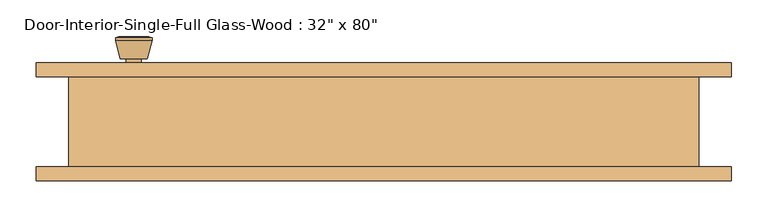
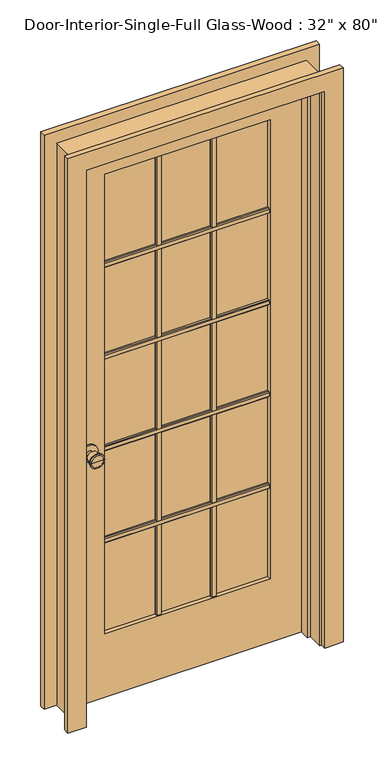
"""IFC4 building model written with IfcOpenShell, lengths in millimetres: door geometry."""

from ifc_helpers import new_model, si_unit, point, frame, frame_2d, origin, place, context, project, spatial, polyline, circle_curve, trimmed, segment, composite_curve, outline, extrude, faceted_brep, source, transform, mapped, element, save
from ifc_brep_helpers import plane_surface, cylinder_surface, revolved_surface, advanced_brep


def door_ad4706cc(model_context):
    return source(origin(), model_context, "Body", "SolidModel", [
        extrude(outline(polyline([(44.7675, 1586.23), (51.1175, 1586.23), (54.2925, 1583.055), (54.2925, 1570.355), (51.1175, 1567.18), (44.7675, 1567.18), (44.7675, 1586.23)])), frame((-285.75, 0.0, 0.0), z_axis=(1.0, 0.0, 0.0), x_axis=(0.0, 1.0, 0.0)), (0.0, 0.0, 1.0), 571.5),
        extrude(outline(polyline([(44.7675, 1249.9975), (51.1175, 1249.9975), (54.2925, 1246.8225), (54.2925, 1234.1225), (51.1175, 1230.9475), (44.7675, 1230.9475), (44.7675, 1249.9975)])), frame((-285.75, 0.0, 0.0), z_axis=(1.0, 0.0, 0.0), x_axis=(0.0, 1.0, 0.0)), (0.0, 0.0, 1.0), 571.5),
        extrude(outline(polyline([(44.7675, 913.765), (51.1175, 913.765), (54.2925, 910.59), (54.2925, 897.89), (51.1175, 894.715), (44.7675, 894.715), (44.7675, 913.765)])), frame((-285.75, 0.0, 0.0), z_axis=(1.0, 0.0, 0.0), x_axis=(0.0, 1.0, 0.0)), (0.0, 0.0, 1.0), 571.5),
        extrude(outline(polyline([(44.7675, 577.5325), (51.1175, 577.5325), (54.2925, 574.3575), (54.2925, 561.6575), (51.1175, 558.4825), (44.7675, 558.4825), (44.7675, 577.5325)])), frame((-285.75, 0.0, 0.0), z_axis=(1.0, 0.0, 0.0), x_axis=(0.0, 1.0, 0.0)), (0.0, 0.0, 1.0), 571.5),
        extrude(outline(polyline([(85.725, 44.7675), (85.725, 51.1175), (88.9, 54.2925), (101.6, 54.2925), (104.775, 51.1175), (104.775, 44.7675), (85.725, 44.7675)])), frame((0.0, 0.0, 231.775), z_axis=(0.0, 0.0, 1.0), x_axis=(1.0, 0.0, 0.0)), (0.0, 0.0, 1.0), 1681.1625),
        extrude(outline(polyline([(-104.775, 44.7675), (-104.775, 51.1175), (-101.6, 54.2925), (-88.9, 54.2925), (-85.725, 51.1175), (-85.725, 44.7675), (-104.775, 44.7675)])), frame((0.0, 0.0, 231.775), z_axis=(0.0, 0.0, 1.0), x_axis=(1.0, 0.0, 0.0)), (0.0, 0.0, 1.0), 1681.1625),
        extrude(outline(polyline([(37.7825, 1586.23), (37.7825, 1567.18), (31.4325, 1567.18), (28.2575, 1570.355), (28.2575, 1583.055), (31.4325, 1586.23), (37.7825, 1586.23)])), frame((-285.75, 0.0, 0.0), z_axis=(1.0, 0.0, 0.0), x_axis=(0.0, 1.0, 0.0)), (0.0, 0.0, 1.0), 571.5),
        extrude(outline(polyline([(37.7825, 1249.9975), (37.7825, 1230.9475), (31.4325, 1230.9475), (28.2575, 1234.1225), (28.2575, 1246.8225), (31.4325, 1249.9975), (37.7825, 1249.9975)])), frame((-285.75, 0.0, 0.0), z_axis=(1.0, 0.0, 0.0), x_axis=(0.0, 1.0, 0.0)), (0.0, 0.0, 1.0), 571.5),
        extrude(outline(polyline([(37.7825, 913.765), (37.7825, 894.715), (31.4325, 894.715), (28.2575, 897.89), (28.2575, 910.59), (31.4325, 913.765), (37.7825, 913.765)])), frame((-285.75, 0.0, 0.0), z_axis=(1.0, 0.0, 0.0), x_axis=(0.0, 1.0, 0.0)), (0.0, 0.0, 1.0), 571.5),
        extrude(outline(polyline([(37.7825, 577.5325), (37.7825, 558.4825), (31.4325, 558.4825), (28.2575, 561.6575), (28.2575, 574.3575), (31.4325, 577.5325), (37.7825, 577.5325)])), frame((-285.75, 0.0, 0.0), z_axis=(1.0, 0.0, 0.0), x_axis=(0.0, 1.0, 0.0)), (0.0, 0.0, 1.0), 571.5),
        extrude(outline(polyline([(85.725, 37.7825), (104.775, 37.7825), (104.775, 31.4325), (101.6, 28.2575), (88.9, 28.2575), (85.725, 31.4325), (85.725, 37.7825)])), frame((0.0, 0.0, 231.775), z_axis=(0.0, 0.0, 1.0), x_axis=(1.0, 0.0, 0.0)), (0.0, 0.0, 1.0), 1681.1625),
        extrude(outline(polyline([(-104.775, 37.7825), (-85.725, 37.7825), (-85.725, 31.4325), (-88.9, 28.2575), (-101.6, 28.2575), (-104.775, 31.4325), (-104.775, 37.7825)])), frame((0.0, 0.0, 231.775), z_axis=(0.0, 0.0, 1.0), x_axis=(1.0, 0.0, 0.0)), (0.0, 0.0, 1.0), 1681.1625),
        advanced_brep(
        [(-342.9, 17.8125, 914.4), (-332.9, 17.8125, 914.4), (-352.9, 17.8125, 914.4), (-322.4241324, -31.1875, 914.4), (-342.9, -31.1875, 914.4), (-363.3758676, -31.1875, 914.4), (-317.9, -29.3596319, 914.4), (-367.9, -29.3596319, 914.4), (-317.9, -25.8959537, 914.4), (-367.9, -25.8959537, 914.4), (-324.263764, -1.1875, 914.4), (-361.536236, -1.1875, 914.4), (-332.9, -1.1875, 914.4), (-352.9, -1.1875, 914.4)],
        [
            (0, 1),
            (1, 2, circle_curve(frame((-342.9, 17.8125, 914.4), z_axis=(0.0, 1.0, 0.0), x_axis=(-1.0, 0.0, 0.0)), 10.0)),
            (2, 0),
            (2, 1, circle_curve(frame((-342.9, 17.8125, 914.4), z_axis=(0.0, 1.0, 0.0), x_axis=(-1.0, 0.0, 0.0)), 10.0)),
            (3, 4),
            (4, 5),
            (5, 3, circle_curve(frame((-342.9, -31.1875, 914.4), z_axis=(0.0, -1.0, 0.0), x_axis=(-1.0, 0.0, 0.0)), 20.4758676)),
            (3, 5, circle_curve(frame((-342.9, -31.1875, 914.4), z_axis=(0.0, -1.0, 0.0), x_axis=(-1.0, 0.0, 0.0)), 20.4758676)),
            (6, 3),
            (5, 7),
            (7, 6, circle_curve(frame((-342.9, -29.3596319, 914.4), z_axis=(0.0, -1.0, 0.0), x_axis=(-1.0, 0.0, 0.0)), 25.0)),
            (6, 7, circle_curve(frame((-342.9, -29.3596319, 914.4), z_axis=(0.0, -1.0, 0.0), x_axis=(-1.0, 0.0, 0.0)), 25.0)),
            (8, 6),
            (7, 9),
            (9, 8, circle_curve(frame((-342.9, -25.8959537, 914.4), z_axis=(0.0, -1.0, 0.0), x_axis=(-1.0, 0.0, 0.0)), 25.0)),
            (8, 9, circle_curve(frame((-342.9, -25.8959537, 914.4), z_axis=(0.0, -1.0, 0.0), x_axis=(-1.0, 0.0, 0.0)), 25.0)),
            (10, 8),
            (9, 11),
            (11, 10, circle_curve(frame((-342.9, -1.1875, 914.4), z_axis=(0.0, -1.0, 0.0), x_axis=(-1.0, 0.0, 0.0)), 18.636236)),
            (10, 11, circle_curve(frame((-342.9, -1.1875, 914.4), z_axis=(0.0, -1.0, 0.0), x_axis=(-1.0, 0.0, 0.0)), 18.636236)),
            (12, 10),
            (11, 13),
            (13, 12, circle_curve(frame((-342.9, -1.1875, 914.4), z_axis=(0.0, -1.0, 0.0), x_axis=(-1.0, 0.0, 0.0)), 10.0)),
            (12, 13, circle_curve(frame((-342.9, -1.1875, 914.4), z_axis=(0.0, -1.0, 0.0), x_axis=(-1.0, 0.0, 0.0)), 10.0)),
            (1, 12),
            (13, 2),
        ],
        [
            plane_surface(frame((-342.9, 17.8125, 914.4), z_axis=(0.0, 1.0, 0.0), x_axis=(-1.0, 0.0, 0.0))),
            plane_surface(frame((-342.9, -31.1875, 914.4), z_axis=(0.0, -1.0, 0.0), x_axis=(-1.0, 0.0, 0.0))),
            revolved_surface(polyline([(-363.3758676, -31.1875, 914.4), (-367.9, -29.3596319, 914.4)]), (-342.9, 17.8125, 914.4), (0.0, 1.0, 0.0)),
            cylinder_surface(frame((-342.9, 17.8125, 914.4), z_axis=(0.0, 1.0, 0.0), x_axis=(-1.0, 0.0, 0.0)), 25.0),
            revolved_surface(polyline([(-367.9, -25.8959537, 914.4), (-361.536236, -1.1875, 914.4)]), (-342.9, 17.8125, 914.4), (0.0, 1.0, 0.0)),
            plane_surface(frame((-342.9, -1.1875, 914.4), z_axis=(0.0, 1.0, 0.0), x_axis=(-1.0, 0.0, 0.0))),
            cylinder_surface(frame((-342.9, 17.8125, 914.4), z_axis=(0.0, 1.0, 0.0), x_axis=(-1.0, 0.0, 0.0)), 10.0),
        ],
        [
            (0, [[1, 2, 3]]),
            (0, [[-3, 4, -1]]),
            (1, [[5, 6, 7]]),
            (1, [[-6, -5, 8]]),
            (2, [[9, -7, 10, 11]]),
            (2, [[-10, -8, -9, 12]]),
            (3, [[13, -11, 14, 15]]),
            (3, [[-14, -12, -13, 16]]),
            (4, [[17, -15, 18, 19]]),
            (4, [[-18, -16, -17, 20]]),
            (5, [[21, -19, 22, 23]]),
            (5, [[-22, -20, -21, 24]]),
            (6, [[25, -23, 26, -2]]),
            (6, [[-26, -24, -25, -4]]),
        ],
    ),
        extrude(outline(composite_curve([segment(trimmed(circle_curve(frame_2d((914.4, -342.9)), 30.0), [point((914.4, -372.9))], [point((914.4, -312.9))], False, "CARTESIAN"), True, "CONTINUOUS"), segment(trimmed(circle_curve(frame_2d((914.4, -342.9)), 30.0), [point((914.4, -312.9))], [point((914.4, -372.9))], False, "CARTESIAN"), True, "CONTINUOUS")], self_intersect=False)), frame((0.0, 17.8125, 0.0), z_axis=(0.0, 1.0, 0.0), x_axis=(0.0, 0.0, 1.0)), (0.0, 0.0, 1.0), 6.0),
        advanced_brep(
        [(-342.9, 64.7375, 914.4), (-352.9, 64.7375, 914.4), (-332.9, 64.7375, 914.4), (-322.4241324, 113.7375, 914.4), (-363.3758676, 113.7375, 914.4), (-342.9, 113.7375, 914.4), (-317.9, 111.9096319, 914.4), (-367.9, 111.9096319, 914.4), (-317.9, 108.4459537, 914.4), (-367.9, 108.4459537, 914.4), (-324.263764, 83.7375, 914.4), (-361.536236, 83.7375, 914.4), (-332.9, 83.7375, 914.4), (-352.9, 83.7375, 914.4)],
        [
            (0, 1),
            (1, 2, circle_curve(frame((-342.9, 64.7375, 914.4), z_axis=(0.0, -1.0, 0.0), x_axis=(-1.0, 0.0, 0.0)), 10.0)),
            (2, 0),
            (2, 1, circle_curve(frame((-342.9, 64.7375, 914.4), z_axis=(0.0, -1.0, 0.0), x_axis=(-1.0, 0.0, 0.0)), 10.0)),
            (3, 4, circle_curve(frame((-342.9, 113.7375, 914.4), z_axis=(0.0, 1.0, 0.0), x_axis=(-1.0, 0.0, 0.0)), 20.4758676)),
            (4, 5),
            (5, 3),
            (4, 3, circle_curve(frame((-342.9, 113.7375, 914.4), z_axis=(0.0, 1.0, 0.0), x_axis=(-1.0, 0.0, 0.0)), 20.4758676)),
            (6, 7, circle_curve(frame((-342.9, 111.9096319, 914.4), z_axis=(0.0, 1.0, 0.0), x_axis=(-1.0, 0.0, 0.0)), 25.0)),
            (7, 4),
            (3, 6),
            (7, 6, circle_curve(frame((-342.9, 111.9096319, 914.4), z_axis=(0.0, 1.0, 0.0), x_axis=(-1.0, 0.0, 0.0)), 25.0)),
            (8, 9, circle_curve(frame((-342.9, 108.4459537, 914.4), z_axis=(0.0, 1.0, 0.0), x_axis=(-1.0, 0.0, 0.0)), 25.0)),
            (9, 7),
            (6, 8),
            (9, 8, circle_curve(frame((-342.9, 108.4459537, 914.4), z_axis=(0.0, 1.0, 0.0), x_axis=(-1.0, 0.0, 0.0)), 25.0)),
            (10, 11, circle_curve(frame((-342.9, 83.7375, 914.4), z_axis=(0.0, 1.0, 0.0), x_axis=(-1.0, 0.0, 0.0)), 18.636236)),
            (11, 9),
            (8, 10),
            (11, 10, circle_curve(frame((-342.9, 83.7375, 914.4), z_axis=(0.0, 1.0, 0.0), x_axis=(-1.0, 0.0, 0.0)), 18.636236)),
            (12, 13, circle_curve(frame((-342.9, 83.7375, 914.4), z_axis=(0.0, 1.0, 0.0), x_axis=(-1.0, 0.0, 0.0)), 10.0)),
            (13, 11),
            (10, 12),
            (13, 12, circle_curve(frame((-342.9, 83.7375, 914.4), z_axis=(0.0, 1.0, 0.0), x_axis=(-1.0, 0.0, 0.0)), 10.0)),
            (1, 13),
            (12, 2),
        ],
        [
            plane_surface(frame((-342.9, 64.7375, 914.4), z_axis=(0.0, -1.0, 0.0), x_axis=(-1.0, 0.0, 0.0))),
            plane_surface(frame((-342.9, 113.7375, 914.4), z_axis=(0.0, 1.0, 0.0), x_axis=(-1.0, 0.0, 0.0))),
            revolved_surface(polyline([(-363.3758676, 113.7375, 914.4), (-367.9, 111.9096319, 914.4)]), (-342.9, 64.7375, 914.4), (0.0, -1.0, 0.0)),
            cylinder_surface(frame((-342.9, 64.7375, 914.4), z_axis=(0.0, -1.0, 0.0), x_axis=(-1.0, 0.0, 0.0)), 25.0),
            revolved_surface(polyline([(-367.9, 108.4459537, 914.4), (-361.536236, 83.7375, 914.4)]), (-342.9, 64.7375, 914.4), (0.0, -1.0, 0.0)),
            plane_surface(frame((-342.9, 83.7375, 914.4), z_axis=(0.0, -1.0, 0.0), x_axis=(-1.0, 0.0, 0.0))),
            cylinder_surface(frame((-342.9, 64.7375, 914.4), z_axis=(0.0, -1.0, 0.0), x_axis=(-1.0, 0.0, 0.0)), 10.0),
        ],
        [
            (0, [[1, 2, 3]]),
            (0, [[-3, 4, -1]]),
            (1, [[5, 6, 7]]),
            (1, [[8, -7, -6]]),
            (2, [[9, 10, -5, 11]]),
            (2, [[12, -11, -8, -10]]),
            (3, [[13, 14, -9, 15]]),
            (3, [[16, -15, -12, -14]]),
            (4, [[17, 18, -13, 19]]),
            (4, [[20, -19, -16, -18]]),
            (5, [[21, 22, -17, 23]]),
            (5, [[24, -23, -20, -22]]),
            (6, [[-2, 25, -21, 26]]),
            (6, [[-4, -26, -24, -25]]),
        ],
    ),
        extrude(outline(composite_curve([segment(trimmed(circle_curve(frame_2d((914.4, -342.9)), 30.0), [point((914.4, -372.9))], [point((914.4, -312.9))], False, "CARTESIAN"), True, "CONTINUOUS"), segment(trimmed(circle_curve(frame_2d((914.4, -342.9)), 30.0), [point((914.4, -312.9))], [point((914.4, -372.9))], False, "CARTESIAN"), True, "CONTINUOUS")], self_intersect=False)), frame((0.0, 58.7375, 0.0), z_axis=(0.0, 1.0, 0.0), x_axis=(0.0, 0.0, 1.0)), (0.0, 0.0, 1.0), 6.0),
        extrude(outline(polyline([(2032.0, -406.4), (0.0, -406.4), (0.0, 406.4), (2032.0, 406.4), (2032.0, -406.4)]), holes=[polyline([(1912.9375, -285.75), (1912.9375, 285.75), (231.775, 285.75), (231.775, -285.75), (1912.9375, -285.75)])]), frame((0.0, 23.8125, 0.0), z_axis=(0.0, 1.0, 0.0), x_axis=(0.0, 0.0, 1.0)), (0.0, 0.0, 1.0), 34.925),
        faceted_brep([(431.8, 58.7375, 0.0), (431.8, -65.0875, 0.0), (406.4, -65.0875, 0.0), (406.4, -11.1125, 0.0), (393.7, -11.1125, 0.0), (393.7, 23.8125, 0.0), (406.4, 23.8125, 0.0), (406.4, 58.7375, 0.0), (431.8, 58.7375, 2057.4), (431.8, -65.0875, 2057.4), (-431.8, -65.0875, 2057.4), (-431.8, -65.0875, 0.0), (-406.4, -65.0875, 0.0), (-406.4, -65.0875, 2032.0), (406.4, -65.0875, 2032.0), (406.4, -11.1125, 2032.0), (-406.4, -11.1125, 2032.0), (-406.4, -11.1125, 0.0), (-393.7, -11.1125, 0.0), (-393.7, -11.1125, 2019.3), (393.7, -11.1125, 2019.3), (393.7, 23.8125, 2019.3), (-393.7, 23.8125, 2019.3), (-393.7, 23.8125, 0.0), (-406.4, 23.8125, 0.0), (-406.4, 23.8125, 2032.0), (406.4, 23.8125, 2032.0), (406.4, 58.7375, 2032.0), (-406.4, 58.7375, 2032.0), (-406.4, 58.7375, 0.0), (-431.8, 58.7375, 0.0), (-431.8, 58.7375, 2057.4)], [[[0, 1, 2, 3, 4, 5, 6, 7]], [[1, 0, 8, 9]], [[2, 1, 9, 10, 11, 12, 13, 14]], [[3, 2, 14, 15]], [[4, 3, 15, 16, 17, 18, 19, 20]], [[5, 4, 20, 21]], [[6, 5, 21, 22, 23, 24, 25, 26]], [[7, 6, 26, 27]], [[0, 7, 27, 28, 29, 30, 31, 8]], [[9, 8, 31, 10]], [[15, 14, 13, 16]], [[21, 20, 19, 22]], [[27, 26, 25, 28]], [[30, 29, 24, 23, 18, 17, 12, 11]], [[10, 31, 30, 11]], [[16, 13, 12, 17]], [[22, 19, 18, 23]], [[28, 25, 24, 29]]]),
        extrude(outline(polyline([(285.75, 37.7825), (-285.75, 37.7825), (-285.75, 44.7675), (285.75, 44.7675), (285.75, 37.7825)])), frame((0.0, 0.0, 231.775), z_axis=(0.0, 0.0, 1.0), x_axis=(1.0, 0.0, 0.0)), (0.0, 0.0, 1.0), 1681.1625),
        extrude(outline(polyline([(0.0, 412.75), (0.0, 476.25), (2101.85, 476.25), (2101.85, -476.25), (0.0, -476.25), (0.0, -412.75), (2038.35, -412.75), (2038.35, 412.75), (0.0, 412.75)])), frame((0.0, -84.1375, 0.0), z_axis=(0.0, 1.0, 0.0), x_axis=(0.0, 0.0, 1.0)), (0.0, 0.0, 1.0), 19.05),
        extrude(outline(polyline([(0.0, 412.75), (0.0, 476.25), (2101.85, 476.25), (2101.85, -476.25), (0.0, -476.25), (0.0, -412.75), (2038.35, -412.75), (2038.35, 412.75), (0.0, 412.75)])), frame((0.0, 58.7375, 0.0), z_axis=(0.0, 1.0, 0.0), x_axis=(0.0, 0.0, 1.0)), (0.0, 0.0, 1.0), 19.05),
    ])


if __name__ == "__main__":
    model = new_model("IFC4")
    model_context = context("Model", 3, world=origin())
    ifc_project = project(units=[si_unit("LENGTHUNIT", "METRE", prefix="MILLI")], contexts=[model_context])
    site = spatial("IfcSite", under=ifc_project)
    building = spatial("IfcBuilding", under=site)
    placement = place(None, origin())
    door_shape = door_ad4706cc(model_context)
    element("IfcDoor", 1, ObjectType="Door-Interior-Single-Full Glass-Wood : 32\" x 80\"", at=placement, inside=building, context=model_context, shape_type="MappedRepresentation", body=[
        mapped(door_shape, transform((0.0, 0.0, 0.0), x_axis=(1.0, 0.0, 0.0), y_axis=(0.0, 1.0, 0.0), z_axis=(0.0, 0.0, 1.0))),
    ])
    save(model, "model.ifc")

# Revit data of these elements
# Type "Door-Interior-Single-Full Glass-Wood : 32\" x 80\""
#   Type Mark = "113"
#   COBie.Type.CreatedBy = "doug.wood@us.ibm.com"
#   COBie.Type.CreatedOn = "2016-04-14T02:07:24"
#   COBie.Type.Name = "Doors_Door-Interior-Single-Full Glass-Wood_32\" x 80\"_113"
#   COBie.Type.Category = "23-30 10 00 : Doors"
#   COBie.Type.Description = "Door-Interior-Single-Full Glass-Wood_32\" x 80\""
#   COBie.Type.Manufacturer = ""
#   COBie.Type.ModelNumber = ""
#   Assembly Code = "C1020300"
#   Analytic Construction = "Wood frame with single clear glass"
#   COBie.Type.ReplacementCost = 0
#   Top Rail = 0' - 4 11/16"
#   Thickness = 0' - 1 3/8"
#   Thermal Resistance (R) = 0.177906 (m²·K)/W
#   Swing Angle [instance default] = 90.00°
#   Stiles = 0' - 4 3/4"
#   Rough Width = 2' - 10"
#   Rough Height = 6' - 9"
#   Height = 6' - 8"
#   Width = 2' - 8"
#   Heat Transfer Coefficient (U) = 5.62148 W/(m²·K)
#   Bottom Rail = 0' - 9 1/8"
#   COBie.Type = no
#   Show Grill [instance default] = yes
#   Trim Material = Trim - White
#   Panel Material = Door - Panel - White
#   Frame Material = Door - Frame - White
#   Door Handle Material = ARCAT - Metal - Brass, Polished
#   Visual Light Transmittance = 0
#   Solar Heat Gain Coefficient = 0
#   Wall Closure = (empty or 0)
#   Function = (empty or 0)
# Element 1 (IfcDoor, "Door-Interior-Single-Full Glass-Wood : 32\" x 80\"")
#   Materials on its faces: "Door - Panel - White", "Aluminum", "Trim - White", "Door - Frame - White", "Glass"
# Materials
#   "Trim - White": class "Wood", colour RGB 255 255 255, transparency 0, Cost = 0
#   "Door - Panel - White": class "Wood", colour RGB 255 255 255, transparency 0, Cost = 0
#   "Door - Frame - White": class "Miscellaneous", colour RGB 255 255 255, transparency 0, Cost = 0
#   "ARCAT - Metal - Brass, Polished": class "Unassigned", colour RGB 246 240 166, transparency 0, Keynote = "05050", Model = "Generic", Manufacturer = "Generic", Description = "Steel, Chrome Plated"
#   "Aluminum": class "Metal", colour RGB 247 247 247, transparency 0, Description = "Aluminum 6061", Cost = 0
#   "Glass": class "Glass", colour RGB 0 128 192, transparency 0.75, Description = "Soda Lime Glass", Cost = 0
